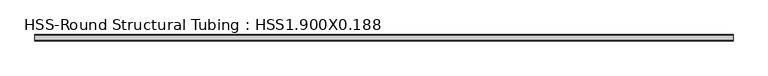
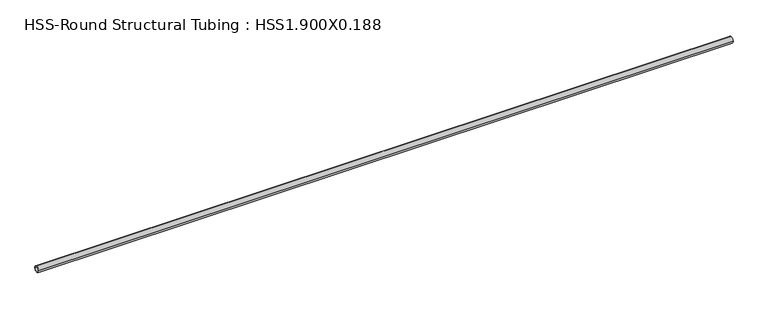
"""IFC4 building model written with IfcOpenShell, lengths in millimetres: member geometry, HSS-Round Structural Tubing : HSS1.900X0.188."""

from ifc_helpers import new_model, si_unit, point, frame, origin, origin_2d, place, context, project, spatial, circle_curve, trimmed, segment, composite_curve, outline, extrude, source, transform, mapped, element, save


def hss_round_structural_tubing_hss1_900x0_188_38155dc2(model_context):
    return source(origin(), model_context, "Body", "SweptSolid", [
        extrude(outline(composite_curve([segment(trimmed(circle_curve(origin_2d(), 24.13), [point((-24.13, 0.0))], [point((24.13, 0.0))], False, "CARTESIAN"), True, "CONTINUOUS"), segment(trimmed(circle_curve(origin_2d(), 24.13), [point((24.13, 0.0))], [point((-24.13, 0.0))], False, "CARTESIAN"), True, "CONTINUOUS")], self_intersect=False), holes=[composite_curve([segment(trimmed(circle_curve(origin_2d(), 19.7104), [point((19.7104, 0.0))], [point((-19.7104, 0.0))], True, "CARTESIAN"), True, "CONTINUOUS"), segment(trimmed(circle_curve(origin_2d(), 19.7104), [point((-19.7104, 0.0))], [point((19.7104, 0.0))], True, "CARTESIAN"), True, "CONTINUOUS")], self_intersect=False)]), frame((-2686.9909377, 0.0, 0.0), z_axis=(1.0, 0.0, 0.0), x_axis=(0.0, 1.0, 0.0)), (0.0, 0.0, 1.0), 5419.0802818),
    ])


if __name__ == "__main__":
    model = new_model("IFC4")
    model_context = context("Model", 3, world=origin())
    ifc_project = project(units=[si_unit("LENGTHUNIT", "METRE", prefix="MILLI")], contexts=[model_context])
    site = spatial("IfcSite", under=ifc_project)
    building = spatial("IfcBuilding", under=site)
    placement = place(None, origin())
    hss_round_structural_tubing_hss1_900x0_188_shape = hss_round_structural_tubing_hss1_900x0_188_38155dc2(model_context)
    element("IfcMember", 1, ObjectType="HSS-Round Structural Tubing : HSS1.900X0.188", at=placement, inside=building, context=model_context, shape_type="MappedRepresentation", body=[
        mapped(hss_round_structural_tubing_hss1_900x0_188_shape, transform((0.0, 0.0, 0.0), x_axis=(1.0, 0.0, 0.0), y_axis=(0.0, 1.0, 0.0), z_axis=(0.0, 0.0, 1.0))),
    ])
    save(model, "model.ifc")

# Revit data of these elements
# Type "HSS-Round Structural Tubing : HSS1.900X0.188"
#   Assembly Code = "B10"
#   t = 4.42 mm
#   W = 3.44
#   Length [instance default] = 1524 mm
#   OD = 48.26 mm
#   A = 0.000608386 m²
#   Structural Material [instance default] = Steel ASTM A500, Grade B, Round
# Element 1 (IfcMember, "HSS-Round Structural Tubing : HSS1.900X0.188")
#   Materials on its faces: "Steel ASTM A500, Grade B, Round"
# Materials
#   "Steel ASTM A500, Grade B, Round": class "Metal", colour RGB 199 199 199, transparency 0, Description = "Carbon steel", Cost = 0
